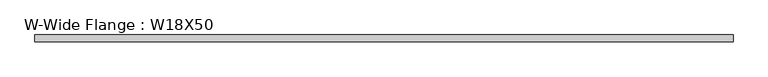
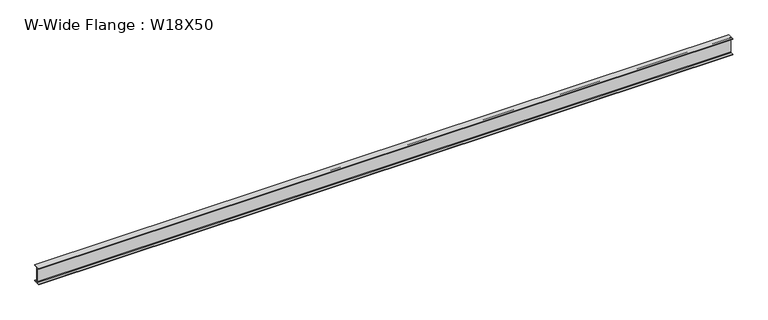
"""IFC4 building model written with IfcOpenShell, lengths in millimetres: beam geometry, W-Wide Flange : W18X50."""

from ifc_helpers import new_model, si_unit, point, frame, frame_2d, origin, place, context, project, spatial, polyline, circle_curve, trimmed, segment, composite_curve, outline, extrude, source, transform, mapped, element, save


def w_wide_flange_w18x50_1414bbc8(model_context):
    return source(origin(), model_context, "Body", "SweptSolid", [
        extrude(outline(composite_curve([segment(polyline([(95.25, -214.122), (95.25, -228.6), (-95.25, -228.6), (-95.25, -214.122), (-21.7805, -214.122)]), True, "CONTINUOUS"), segment(trimmed(circle_curve(frame_2d((-21.7805, -196.85)), 17.272), [point((-21.7805, -214.122))], [point((-4.5085, -196.85))], True, "CARTESIAN"), True, "CONTINUOUS"), segment(polyline([(-4.5085, -196.85), (-4.5085, 196.85)]), True, "CONTINUOUS"), segment(trimmed(circle_curve(frame_2d((-21.7805, 196.85)), 17.272), [point((-4.5085, 196.85))], [point((-21.7805, 214.122))], True, "CARTESIAN"), True, "CONTINUOUS"), segment(polyline([(-21.7805, 214.122), (-95.25, 214.122), (-95.25, 228.6), (95.25, 228.6), (95.25, 214.122), (21.7805, 214.122)]), True, "CONTINUOUS"), segment(trimmed(circle_curve(frame_2d((21.7805, 196.85)), 17.272), [point((21.7805, 214.122))], [point((4.5085, 196.85))], True, "CARTESIAN"), True, "CONTINUOUS"), segment(polyline([(4.5085, 196.85), (4.5085, -196.85)]), True, "CONTINUOUS"), segment(trimmed(circle_curve(frame_2d((21.7805, -196.85)), 17.272), [point((4.5085, -196.85))], [point((21.7805, -214.122))], True, "CARTESIAN"), True, "CONTINUOUS"), segment(polyline([(21.7805, -214.122), (95.25, -214.122)]), True, "CONTINUOUS")], self_intersect=False)), frame((-9518.65, 0.0, 0.0), z_axis=(1.0, 0.0, 0.0), x_axis=(0.0, 1.0, 0.0)), (0.0, 0.0, 1.0), 18931.89),
    ])


if __name__ == "__main__":
    model = new_model("IFC4")
    model_context = context("Model", 3, world=origin())
    ifc_project = project(units=[si_unit("LENGTHUNIT", "METRE", prefix="MILLI")], contexts=[model_context])
    site = spatial("IfcSite", under=ifc_project)
    building = spatial("IfcBuilding", under=site)
    placement = place(None, origin())
    w_wide_flange_w18x50_shape = w_wide_flange_w18x50_1414bbc8(model_context)
    element("IfcBeam", 1, ObjectType="W-Wide Flange : W18X50", at=placement, inside=building, context=model_context, shape_type="MappedRepresentation", body=[
        mapped(w_wide_flange_w18x50_shape, transform((0.0, 0.0, 0.0), x_axis=(1.0, 0.0, 0.0), y_axis=(0.0, 1.0, 0.0), z_axis=(0.0, 0.0, 1.0))),
    ])
    save(model, "model.ifc")

# Revit data of these elements
# Type "W-Wide Flange : W18X50"
#   Assembly Code = "B10"
#   W = 50
#   Length [instance default] = 5' - 0"
#   bf = 0' - 7 1/2"
#   d = 1' - 6"
#   k = 0' - 1 1/4"
#   k2 = 0' - 0.68"
#   tf = 0' - 0.57"
#   tw = 0' - 0.355"
#   A = 0.102083 SF
#   Structural Material [instance default] = Steel ASTM A992
# Element 1 (IfcBeam, "W-Wide Flange : W18X50")
#   Structural Material = Steel ASTM A36
#   Materials on its faces: "Steel ASTM A36"
# Materials
#   "Steel ASTM A992": class "Metal", colour RGB 199 199 199, transparency 0, Description = "Structural steel 50ksi", Cost = 0
#   "Steel ASTM A36": class "Metal", colour RGB 199 199 199, transparency 0, Description = "Structural steel, ASTM A36 Grade B, mill finish", Cost = 0
